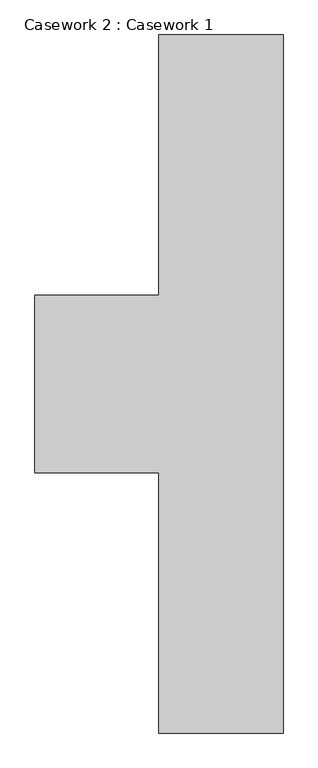
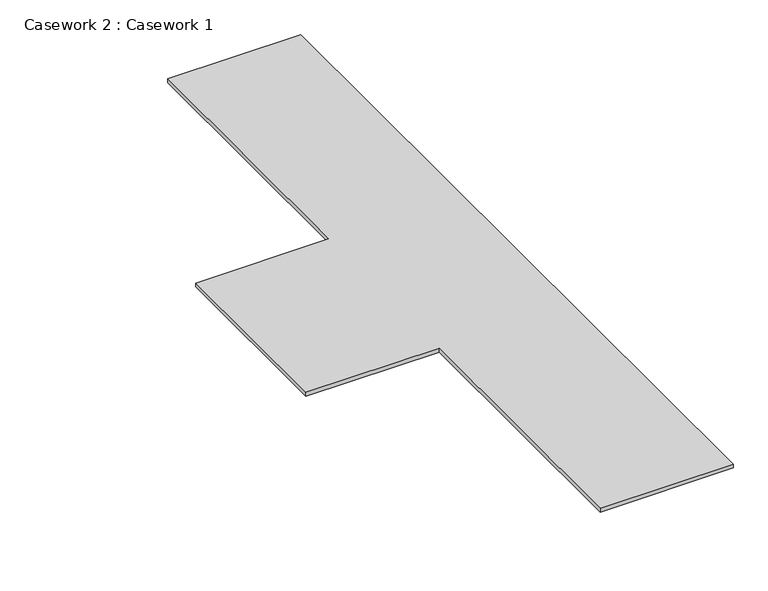
"""IFC4 building model written with IfcOpenShell, lengths in millimetres: furniture geometry, Casework 2 : Casework 1."""

from ifc_helpers import new_model, si_unit, frame, origin, place, context, project, spatial, polyline, outline, extrude, source, transform, mapped, element, save


def casework_2_casework_1_26c335f7(model_context):
    return source(origin(), model_context, "Body", "SweptSolid", [
        extrude(outline(polyline([(46964.5996124, 38594.4930725), (46964.5996124, 40378.8434601), (47815.5, 40378.8434601), (47815.5, 35590.9426849), (46964.5996124, 35590.9426849), (46964.5996124, 37375.2930725), (46113.7003876, 37375.2930725), (46113.7003876, 38594.4930725), (46964.5996124, 38594.4930725)])), frame((0.0, 0.0, 736.6), z_axis=(0.0, 0.0, 1.0), x_axis=(1.0, 0.0, 0.0)), (0.0, 0.0, 1.0), 25.4),
    ])


if __name__ == "__main__":
    model = new_model("IFC4")
    model_context = context("Model", 3, world=origin())
    ifc_project = project(units=[si_unit("LENGTHUNIT", "METRE", prefix="MILLI")], contexts=[model_context])
    site = spatial("IfcSite", under=ifc_project)
    building = spatial("IfcBuilding", under=site)
    placement = place(None, origin())
    casework_2_casework_1_shape = casework_2_casework_1_26c335f7(model_context)
    element("IfcFurniture", 1, ObjectType="Casework 2 : Casework 1", at=placement, inside=building, context=model_context, shape_type="MappedRepresentation", body=[
        mapped(casework_2_casework_1_shape, transform((0.0, 0.0, 0.0), x_axis=(1.0, 0.0, 0.0), y_axis=(0.0, 1.0, 0.0), z_axis=(0.0, 0.0, 1.0))),
    ])
    save(model, "model.ifc")

# Revit data of these elements
# Element 1 (IfcFurniture, "Casework 2 : Casework 1")
#   Materials on its faces: "EXISTING WORKSTATION"
# Materials
#   "EXISTING WORKSTATION": class "Generic", colour RGB 120 120 120, transparency 0, Cost = 0
